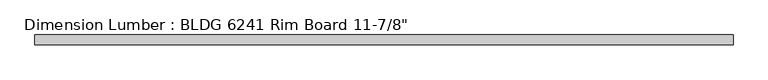
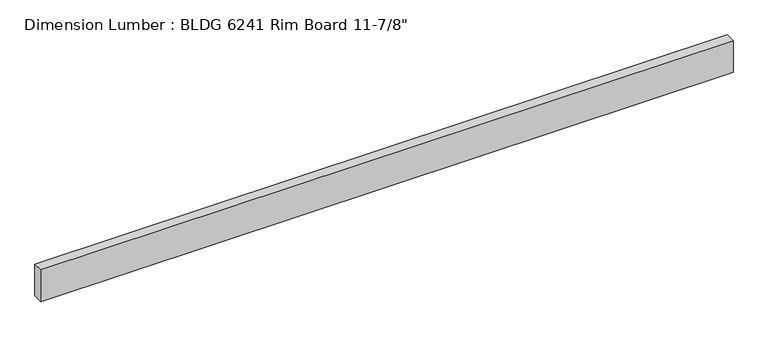
"""IFC4 building model written with IfcOpenShell, lengths in millimetres: beam geometry."""

from ifc_helpers import new_model, si_unit, frame, origin, place, context, project, spatial, polyline, outline, extrude, source, transform, mapped, element, save


def beam_51e41891(model_context):
    return source(origin(), model_context, "Body", "SweptSolid", [
        extrude(outline(polyline([(3159.125, 44.45), (3159.125, -44.45), (-3070.225, -44.45), (-3070.225, 44.45), (3159.125, 44.45)])), frame((0.0, 0.0, -150.8125), z_axis=(0.0, 0.0, 1.0), x_axis=(1.0, 0.0, 0.0)), (0.0, 0.0, 1.0), 301.625),
    ])


if __name__ == "__main__":
    model = new_model("IFC4")
    model_context = context("Model", 3, world=origin())
    ifc_project = project(units=[si_unit("LENGTHUNIT", "METRE", prefix="MILLI")], contexts=[model_context])
    site = spatial("IfcSite", under=ifc_project)
    building = spatial("IfcBuilding", under=site)
    placement = place(None, origin())
    beam_shape = beam_51e41891(model_context)
    element("IfcBeam", 1, ObjectType="Dimension Lumber : BLDG 6241 Rim Board 11-7/8\"", at=placement, inside=building, context=model_context, shape_type="MappedRepresentation", body=[
        mapped(beam_shape, transform((0.0, 0.0, 0.0), x_axis=(1.0, 0.0, 0.0), y_axis=(0.0, 1.0, 0.0), z_axis=(0.0, 0.0, 1.0))),
    ])
    save(model, "model.ifc")

# Revit data of these elements
# Type "Dimension Lumber : BLDG 6241 Rim Board 11-7/8\""
#   Assembly Code = "B10"
#   A = 0.273472 SF
#   Length [instance default] = 5' - 0"
#   b = 0' - 3 1/2"
#   d = 0' - 11 7/8"
#   Structural Material [instance default] = Softwood, Lumber
# Element 1 (IfcBeam, "Dimension Lumber : BLDG 6241 Rim Board 11-7/8\"")
#   Materials on its faces: "Softwood, Lumber"
# Materials
#   "Softwood, Lumber": class "Wood", colour RGB 223 192 134, transparency 0, Description = "Pinus Echinata", Cost = 0
